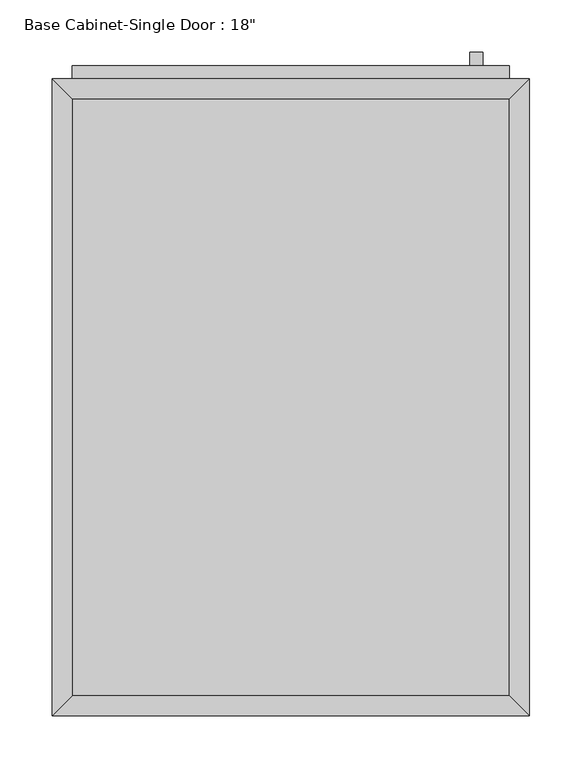
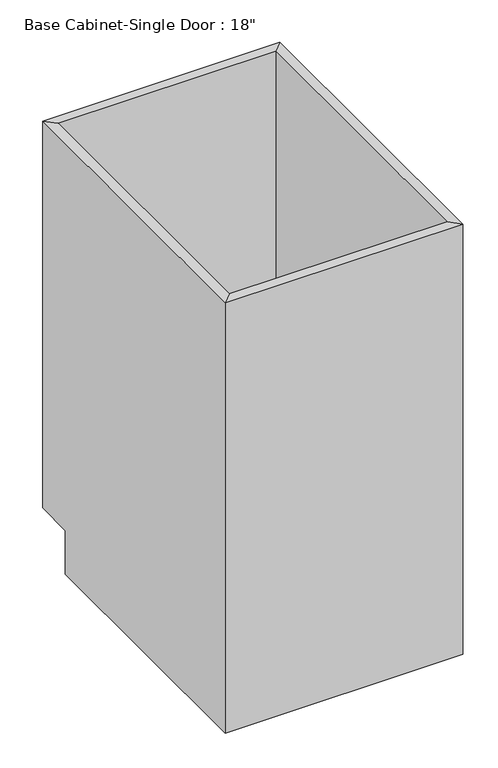
"""IFC4 building model written with IfcOpenShell, lengths in millimetres: furniture geometry."""

from ifc_helpers import new_model, si_unit, frame, origin, place, context, project, spatial, polyline, outline, extrude, faceted_brep, source, transform, mapped, element, save


def furniture_f69173f2(model_context):
    return source(origin(), model_context, "Body", "SolidModel", [
        faceted_brep([(228.2877049, 590.55, 876.3), (-190.8122951, 590.55, 876.3), (-190.8122951, 590.55, 88.9), (228.2877049, 590.55, 88.9), (247.3377049, 609.6, 876.3), (-209.8622951, 609.6, 876.3), (247.3377049, 609.6, 88.9), (-209.8622951, 609.6, 88.9), (-190.8122951, 19.05, 876.3), (-190.8122951, 19.05, 88.9), (-190.8122951, 533.4, 88.9), (-209.8622951, 0.0, 876.3), (-209.8622951, 533.4, 88.9), (-209.8622951, 533.4, 0.0), (-209.8622951, 0.0, 0.0), (228.2877049, 19.05, 876.3), (228.2877049, 19.05, 88.9), (247.3377049, 0.0, 876.3), (247.3377049, 0.0, 0.0), (228.2877049, 533.4, 88.9), (247.3377049, 533.4, 0.0), (247.3377049, 533.4, 88.9)], [[[0, 1, 2, 3]], [[0, 4, 5, 1]], [[4, 6, 7, 5]], [[2, 7, 6, 3]], [[1, 8, 9, 10, 2]], [[5, 11, 8, 1]], [[7, 12, 13, 14, 11, 5]], [[2, 10, 12, 7]], [[8, 15, 16, 9]], [[11, 17, 15, 8]], [[14, 18, 17, 11]], [[3, 19, 16, 15, 0]], [[0, 15, 17, 4]], [[4, 17, 18, 20, 21, 6]], [[6, 21, 19, 3]], [[10, 9, 16, 19]], [[18, 14, 13, 20]], [[13, 12, 10, 19, 21, 20]]]),
        extrude(outline(polyline([(228.2877049, 19.05), (-190.8122951, 19.05), (-190.8122951, 590.55), (228.2877049, 590.55), (228.2877049, 19.05)])), frame((0.0, 0.0, 88.9), z_axis=(0.0, 0.0, 1.0), x_axis=(1.0, 0.0, 0.0)), (0.0, 0.0, 1.0), 19.05),
        extrude(outline(polyline([(202.8877049, 635.0), (202.8877049, 622.3), (190.1877049, 622.3), (190.1877049, 635.0), (202.8877049, 635.0)])), frame((0.0, 0.0, 717.55), z_axis=(0.0, 0.0, 1.0), x_axis=(1.0, 0.0, 0.0)), (0.0, 0.0, 1.0), 101.6),
        extrude(outline(polyline([(228.2877049, 622.3), (228.2877049, 609.6), (-190.8122951, 609.6), (-190.8122951, 622.3), (228.2877049, 622.3)])), frame((0.0, 0.0, 107.95), z_axis=(0.0, 0.0, 1.0), x_axis=(1.0, 0.0, 0.0)), (0.0, 0.0, 1.0), 749.3),
    ])


if __name__ == "__main__":
    model = new_model("IFC4")
    model_context = context("Model", 3, world=origin())
    ifc_project = project(units=[si_unit("LENGTHUNIT", "METRE", prefix="MILLI")], contexts=[model_context])
    site = spatial("IfcSite", under=ifc_project)
    building = spatial("IfcBuilding", under=site)
    placement = place(None, origin())
    furniture_shape = furniture_f69173f2(model_context)
    element("IfcFurniture", 1, ObjectType="Base Cabinet-Single Door : 18\"", at=placement, inside=building, context=model_context, shape_type="MappedRepresentation", body=[
        mapped(furniture_shape, transform((0.0, 0.0, 0.0), x_axis=(1.0, 0.0, 0.0), y_axis=(0.0, 1.0, 0.0), z_axis=(0.0, 0.0, 1.0))),
    ])
    save(model, "model.ifc")

# Revit data of these elements
# Type "Base Cabinet-Single Door : 18\""
#   Assembly Code = "C1030410"
#   Depth = 2' - 0"
#   Height = 2' - 10 1/2"
#   Toe Depth = 0' - 3"
#   Toe Height = 0' - 3 1/2"
#   Width = 1' - 6"
#   Cabinet Material = Countertop & Shelf
#   Drawer Material = Countertop & Shelf
#   Handle Material = Cabinets - Handles
# Element 1 (IfcFurniture, "Base Cabinet-Single Door : 18\"")
#   Materials on its faces: "Countertop & Shelf", "Cabinets", "Cabinets - Handles"
# Materials
#   "Countertop & Shelf": class "Paint", colour RGB 76 54 29, transparency 0, Cost = 0
#   "Cabinets - Handles": class "Metal", colour RGB 57 57 57, transparency 0
#   "Cabinets": class "Miscellaneous", colour RGB 249 249 249, transparency 0
